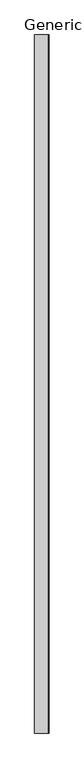
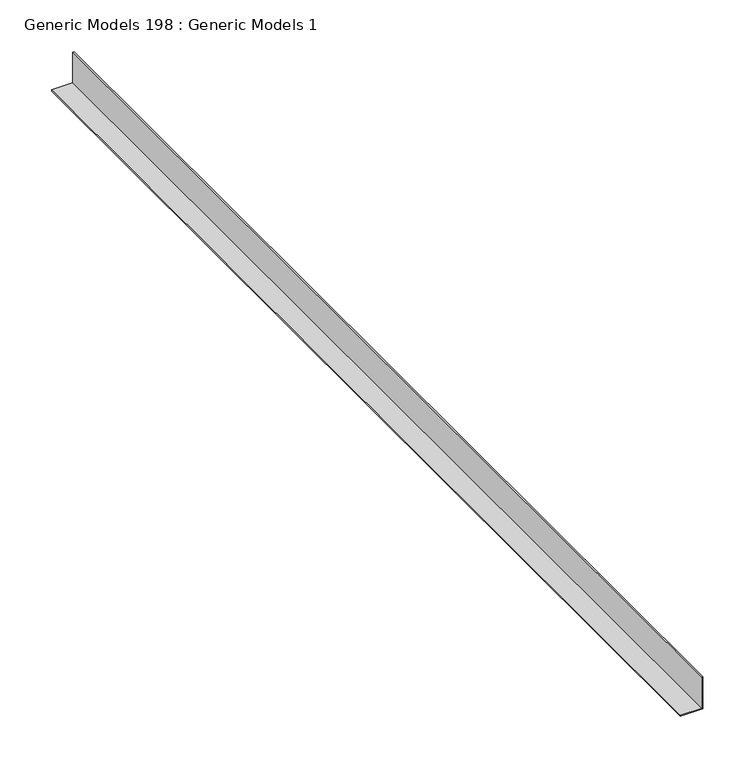
"""IFC4 building model written with IfcOpenShell, lengths in millimetres: proxy geometry, Generic Models 198 : Generic Models 1."""

from ifc_helpers import new_model, si_unit, frame, origin, place, context, project, spatial, polyline, outline, extrude, source, transform, mapped, element, save


def generic_models_198_generic_models_1_f99cc74d(model_context):
    return source(origin(), model_context, "Body", "SweptSolid", [
        extrude(outline(polyline([(2277.1204978, 49676.05), (2277.1204978, 49674.4625), (2240.6079978, 49674.4625), (2240.6079978, 49650.65), (2239.0204978, 49650.65), (2239.0204978, 49676.05), (2277.1204978, 49676.05)])), frame((0.0, 0.0, 0.0), z_axis=(0.0, 1.0, 0.0), x_axis=(0.0, 0.0, 1.0)), (0.0, 0.0, 1.0), 1219.2),
    ])


if __name__ == "__main__":
    model = new_model("IFC4")
    model_context = context("Model", 3, world=origin())
    ifc_project = project(units=[si_unit("LENGTHUNIT", "METRE", prefix="MILLI")], contexts=[model_context])
    site = spatial("IfcSite", under=ifc_project)
    building = spatial("IfcBuilding", under=site)
    placement = place(None, origin())
    generic_models_198_generic_models_1_shape = generic_models_198_generic_models_1_f99cc74d(model_context)
    element("IfcBuildingElementProxy", 1, Name="Generic Models 198 : Generic Models 1", ObjectType="Generic Models 198 : Generic Models 1", at=placement, inside=building, context=model_context, shape_type="MappedRepresentation", body=[
        mapped(generic_models_198_generic_models_1_shape, transform((0.0, 0.0, 0.0), x_axis=(1.0, 0.0, 0.0), y_axis=(0.0, 1.0, 0.0), z_axis=(0.0, 0.0, 1.0))),
    ])
    save(model, "model.ifc")

# Revit data of these elements
# Element 1 (IfcBuildingElementProxy, "Generic Models 198 : Generic Models 1")
#   Materials on its faces: "CEILING TRACK AS SCHEDULED"
# Materials
#   "CEILING TRACK AS SCHEDULED": class "Unassigned", colour RGB 210 209 208, transparency 0, Keynote = "M05121300.02", Cost = 0
